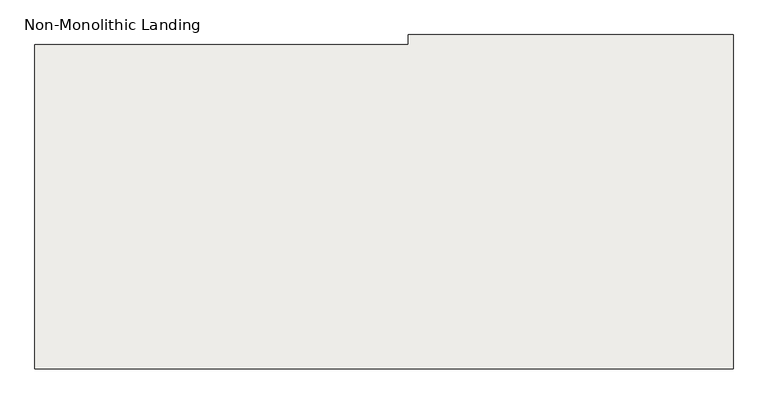
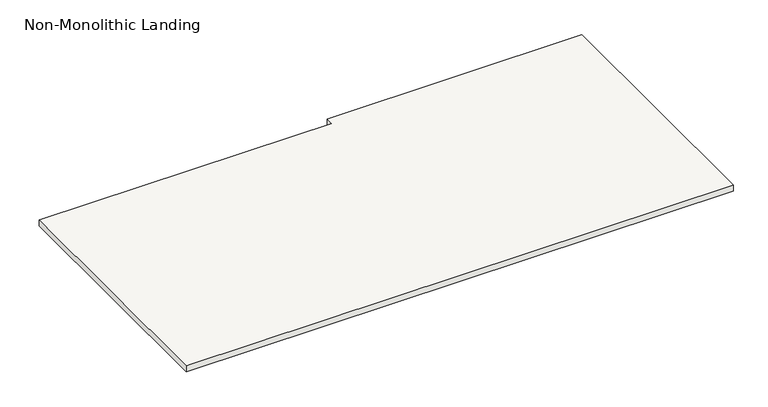
"""IFC4 building model written with IfcOpenShell, lengths in millimetres: slab geometry, Non-Monolithic Landing."""

from ifc_helpers import new_model, si_unit, frame, origin, place, context, project, spatial, polyline, outline, extrude, source, transform, mapped, element, save


def non_monolithic_landing_e847aa32(model_context):
    return source(origin(), model_context, "Body", "SweptSolid", [
        extrude(outline(polyline([(17000.0002442, 21429.9999999), (17000.0002442, 19369.9999999), (12700.0002443, 19369.9999999), (12700.0002443, 21369.9999999), (14700.0002443, 21369.9999999), (15000.0002442, 21369.9999999), (15000.0002442, 21429.9999999), (17000.0002442, 21429.9999999)])), frame((0.0, 0.0, 23616.6666667), z_axis=(0.0, 0.0, 1.0), x_axis=(1.0, 0.0, 0.0)), (0.0, 0.0, 1.0), 50.0),
    ])


if __name__ == "__main__":
    model = new_model("IFC4")
    model_context = context("Model", 3, world=origin())
    ifc_project = project(units=[si_unit("LENGTHUNIT", "METRE", prefix="MILLI")], contexts=[model_context])
    site = spatial("IfcSite", under=ifc_project)
    building = spatial("IfcBuilding", under=site)
    placement = place(None, origin())
    non_monolithic_landing_shape = non_monolithic_landing_e847aa32(model_context)
    element("IfcSlab", 1, ObjectType="Non-Monolithic Landing", at=placement, inside=building, context=model_context, shape_type="MappedRepresentation", body=[
        mapped(non_monolithic_landing_shape, transform((0.0, 0.0, 0.0), x_axis=(1.0, 0.0, 0.0), y_axis=(0.0, 1.0, 0.0), z_axis=(0.0, 0.0, 1.0))),
    ])
    save(model, "model.ifc")
